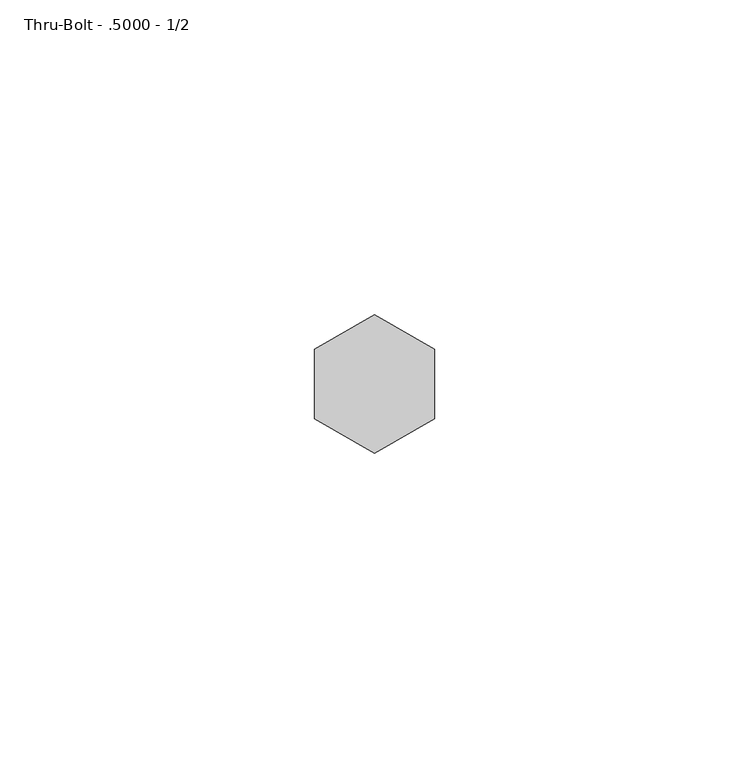
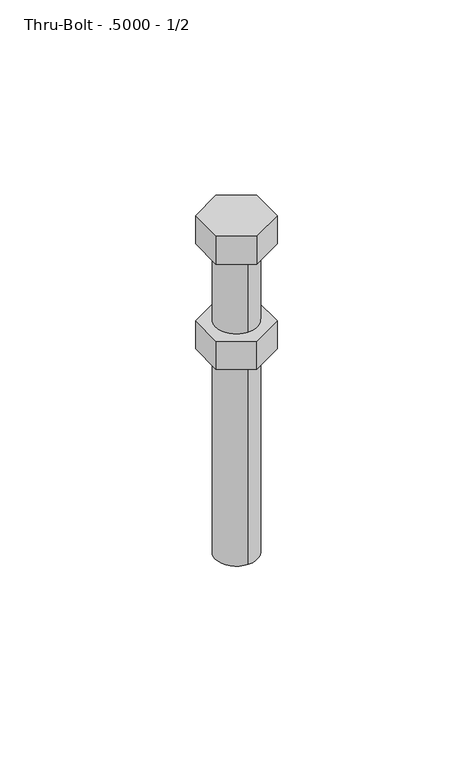
"""IFC4 building model written with IfcOpenShell, lengths in millimetres: fastener geometry, 060523 - W_P_C - Fastenings - Generic : Thru-Bolt - .5000 - 1/2."""

from ifc_helpers import new_model, si_unit, point, frame, origin, origin_with_axes, origin_2d, place, context, project, spatial, polyline, circle_curve, trimmed, segment, composite_curve, outline, extrude, source, transform, mapped, element, save


def thru_bolt_5000_1_2_58b1e949(model_context):
    return source(origin(), model_context, "Body", "SweptSolid", [
        extrude(outline(polyline([(-9.525, -5.4992613), (-9.525, 5.4992613), (0.0, 10.9985226), (9.525, 5.4992613), (9.525, -5.4992613), (0.0, -10.9985226), (-9.525, -5.4992613)])), frame((0.0, 0.0, -34.6273438), z_axis=(0.0, 0.0, 1.0), x_axis=(1.0, 0.0, 0.0)), (0.0, 0.0, 1.0), 9.2273437),
        extrude(outline(polyline([(-9.525, 5.4992613), (0.0, 10.9985226), (9.525, 5.4992613), (9.525, -5.4992613), (0.0, -10.9985226), (-9.525, -5.4992613), (-9.525, 5.4992613)])), origin_with_axes(), (0.0, 0.0, 1.0), 9.2273437),
        extrude(outline(composite_curve([segment(trimmed(circle_curve(origin_2d(), 6.5484375), [point((0.0, -6.5484375))], [point((0.0, 6.5484375))], False, "CARTESIAN"), True, "CONTINUOUS"), segment(trimmed(circle_curve(origin_2d(), 6.5484375), [point((0.0, 6.5484375))], [point((0.0, -6.5484375))], False, "CARTESIAN"), True, "CONTINUOUS")], self_intersect=False)), frame((0.0, 0.0, -101.6), z_axis=(0.0, 0.0, 1.0), x_axis=(1.0, 0.0, 0.0)), (0.0, 0.0, 1.0), 101.6),
    ])


if __name__ == "__main__":
    model = new_model("IFC4")
    model_context = context("Model", 3, world=origin())
    ifc_project = project(units=[si_unit("LENGTHUNIT", "METRE", prefix="MILLI")], contexts=[model_context])
    site = spatial("IfcSite", under=ifc_project)
    building = spatial("IfcBuilding", under=site)
    placement = place(None, origin())
    thru_bolt_5000_1_2_shape = thru_bolt_5000_1_2_58b1e949(model_context)
    element("IfcFastener", 1, ObjectType="060523 - W_P_C - Fastenings - Generic : Thru-Bolt - .5000 - 1/2", at=placement, inside=building, context=model_context, shape_type="MappedRepresentation", body=[
        mapped(thru_bolt_5000_1_2_shape, transform((0.0, 0.0, 0.0), x_axis=(1.0, 0.0, 0.0), y_axis=(0.0, 1.0, 0.0), z_axis=(0.0, 0.0, 1.0))),
    ])
    save(model, "model.ifc")

# Revit data of these elements
# Type "060523 - W_P_C - Fastenings - Generic : Thru-Bolt - .5000 - 1/2"
#   Washer_Thickness = 0' - 0 31/256"
#   Washer Radius = 0' - 0 159/256"
#   Washer Offset - Head = 0' - 0"
#   Washer Offset = 0' - 0"
#   Thickness_of_Substrate [instance default] = 0' - 1"
#   Side = 0' - 0 111/256"
#   Radius = 0' - 0 33/128"
#   Length [instance default] = 0' - 4"
#   Head Size = 0' - 0 3/4"
#   Head Radius = 0' - 0 3/8"
#   Head Height = 0' - 0 93/256"
#   Double Diameter = 0' - 1 1/32"
#   Diameter = 0' - 0 33/64"
#   Default Elevation = 4' - 0"
#   Washer_Nut_Visibility = no
#   Washer_Head_Visibility = no
#   Round_Head_Visibility = no
#   Point Visibility = no
#   Nut_Visibility = yes
#   Hex_Head_Visiblilty = yes
#   Washer Material = none
#   Bolt Material (Size) = AT SILL - FASTENER AT 24" O.C.
# Element 1 (IfcFastener, "060523 - W_P_C - Fastenings - Generic : Thru-Bolt - .5000 - 1/2")
#   Materials on its faces: "AT SILL - FASTENER AT 24\" O.C."
# Materials
#   "AT SILL - FASTENER AT 24\" O.C.": class "Generic", colour RGB 120 120 120, transparency 0, Cost = 0
